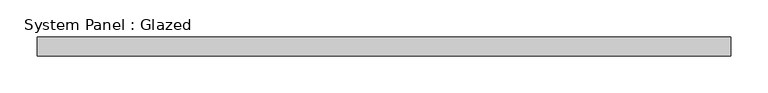
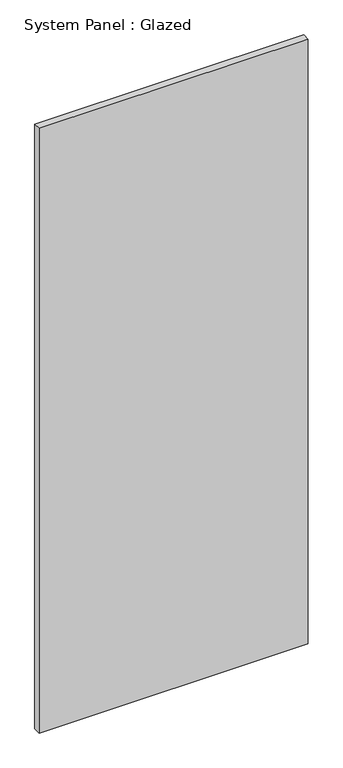
"""IFC4 building model written with IfcOpenShell, lengths in millimetres: plate geometry, System Panel : Glazed."""

import ifcopenshell
import ifcopenshell.guid

model = None  # the IFC model being written
_history = None  # IfcOwnerHistory: only IFC2X3 demands one
_inside = {}  # id of a spatial element -> (the spatial element, [elements in it])
_under = {}  # id of a project, library or spatial element -> (it, [spatial elements below it])
_declared = {}  # id of a project -> (the project, [libraries it declares])
_typed = {}  # id of a type object -> (the type object, [elements of that type])
_made_of = {}  # id of a material, layer set ... -> (it, [elements and type objects made of it])


def new_model(schema):
    """Start an empty IFC model of exactly this schema.

    Asked for "IFC4X3", IfcOpenShell would pick the latest addendum, in which some entities
    have other attributes; the version numbers below select the first issue.
    IFC2X3 requires an IfcOwnerHistory on every rooted entity: one is made here for all.
    """
    global model, _history
    if schema == "IFC4X3":
        model = ifcopenshell.file(schema_version=(4, 3, 0, 0))
    else:
        model = ifcopenshell.file(schema=schema)
    _inside.clear()
    _under.clear()
    _declared.clear()
    _typed.clear()
    _made_of.clear()
    _history = None
    if model.schema == "IFC2X3":
        org = make("IfcOrganization", Name="unknown")
        user = make(
            "IfcPersonAndOrganization",
            ThePerson=make("IfcPerson", FamilyName="unknown"),
            TheOrganization=org,
        )
        app = make(
            "IfcApplication",
            ApplicationDeveloper=org,
            Version="unknown",
            ApplicationFullName="unknown",
            ApplicationIdentifier="unknown",
        )
        _history = make(
            "IfcOwnerHistory",
            OwningUser=user,
            OwningApplication=app,
            ChangeAction="ADDED",
            CreationDate=0,
        )
    return model


def make(cls, **values):
    """One entity of the class cls with the attributes given. An attribute that is None is left unset."""
    return model.create_entity(
        cls, **{name: value for name, value in values.items() if value is not None}
    )


def rooted(cls, **values):
    """An entity with a GlobalId (a new one), such as an element, a storey or a relation."""
    return make(cls, GlobalId=ifcopenshell.guid.new(), OwnerHistory=_history, **values)


def si_unit(unit_type, name, prefix=None):
    """IfcSIUnit, for example si_unit("LENGTHUNIT", "METRE", prefix="MILLI")."""
    return make("IfcSIUnit", UnitType=unit_type, Prefix=prefix, Name=name)


def assignment(units):
    """IfcUnitAssignment: the units of a project."""
    return None if units is None else make("IfcUnitAssignment", Units=units)


def point(xyz):
    """IfcCartesianPoint."""
    return None if xyz is None else make("IfcCartesianPoint", Coordinates=xyz)


def direction(xyz):
    """IfcDirection."""
    return None if xyz is None else make("IfcDirection", DirectionRatios=xyz)


def frame(location, z_axis=None, x_axis=None):
    """IfcAxis2Placement3D, a coordinate frame: its origin and axes. An axis left out is left unset."""
    return make(
        "IfcAxis2Placement3D",
        Location=point(location),
        Axis=direction(z_axis),
        RefDirection=direction(x_axis),
    )


def origin():
    """The frame at (0, 0, 0) with its axes left unset."""
    return frame((0.0, 0.0, 0.0))


def origin_with_axes():
    """The frame at (0, 0, 0) with the z axis (0, 0, 1) and the x axis (1, 0, 0) written out."""
    return frame((0.0, 0.0, 0.0), z_axis=(0.0, 0.0, 1.0), x_axis=(1.0, 0.0, 0.0))


def place(relative_to, where):
    """IfcLocalPlacement: puts the frame where relative to a parent placement (None: the world)."""
    return make(
        "IfcLocalPlacement", PlacementRelTo=relative_to, RelativePlacement=where
    )


def context(
    kind, dimensions, precision=None, world=None, true_north=None, identifier=None
):
    """IfcGeometricRepresentationContext, for example the 3D "Model" context."""
    return make(
        "IfcGeometricRepresentationContext",
        ContextIdentifier=identifier,
        ContextType=kind,
        CoordinateSpaceDimension=dimensions,
        Precision=precision,
        WorldCoordinateSystem=world,
        TrueNorth=true_north,
    )


def project(units=None, contexts=None):
    """IfcProject with its units and contexts."""
    return rooted(
        "IfcProject",
        Name="project",
        RepresentationContexts=contexts,
        UnitsInContext=assignment(units),
    )


def spatial(cls, under=None, at=None, **own):
    """A site, building, storey or space (cls), placed at a placement, below another one or the project."""
    s = rooted(cls, ObjectPlacement=at, **own)
    if under is not None:
        _under.setdefault(under.id(), (under, []))[1].append(s)
    return s


def polyline(points):
    """IfcPolyline through the points."""
    return make("IfcPolyline", Points=[point(p) for p in points])


def outline(outer, holes=None, kind="AREA"):
    """IfcArbitraryClosedProfileDef: a profile drawn as a closed curve; with holes, ...WithVoids."""
    if holes is None:
        return make("IfcArbitraryClosedProfileDef", ProfileType=kind, OuterCurve=outer)
    return make(
        "IfcArbitraryProfileDefWithVoids",
        ProfileType=kind,
        OuterCurve=outer,
        InnerCurves=holes,
    )


def extrude(swept, where, along, depth):
    """IfcExtrudedAreaSolid: the profile swept, set in the frame where, extruded along a direction by depth."""
    return make(
        "IfcExtrudedAreaSolid",
        SweptArea=swept,
        Position=where,
        ExtrudedDirection=direction(along),
        Depth=depth,
    )


def shape(context_of_items, identifier, shape_type, items):
    """IfcShapeRepresentation: the items that make up one representation, for example the "Body"."""
    return make(
        "IfcShapeRepresentation",
        ContextOfItems=context_of_items,
        RepresentationIdentifier=identifier,
        RepresentationType=shape_type,
        Items=items,
    )


def source(mapping_origin, context_of_items, identifier, shape_type, items):
    """IfcRepresentationMap: a shape defined once, which mapped items show again and again."""
    return make(
        "IfcRepresentationMap",
        MappingOrigin=mapping_origin,
        MappedRepresentation=shape(context_of_items, identifier, shape_type, items),
    )


def transform(
    local_origin,
    x_axis=None,
    y_axis=None,
    z_axis=None,
    scale=None,
    scale2=None,
    scale3=None,
    uniform=True,
):
    """IfcCartesianTransformationOperator3D, or its non-uniform kind. x_axis, y_axis, z_axis: its Axis1, 2, 3."""
    if uniform:
        return make(
            "IfcCartesianTransformationOperator3D",
            Axis1=direction(x_axis),
            Axis2=direction(y_axis),
            LocalOrigin=point(local_origin),
            Scale=scale,
            Axis3=direction(z_axis),
        )
    return make(
        "IfcCartesianTransformationOperator3DnonUniform",
        Axis1=direction(x_axis),
        Axis2=direction(y_axis),
        LocalOrigin=point(local_origin),
        Scale=scale,
        Axis3=direction(z_axis),
        Scale2=scale2,
        Scale3=scale3,
    )


def mapped(mapping_source, mapping_target):
    """IfcMappedItem: shows the shape of a source again, moved by a transform."""
    return make(
        "IfcMappedItem", MappingSource=mapping_source, MappingTarget=mapping_target
    )


def made_of(thing, what):
    """Note that an element or type object is made of a material, layer set ...; save() writes the relation."""
    if what is not None:
        _made_of.setdefault(what.id(), (what, []))[1].append(thing)
    return thing


def element(
    cls,
    number,
    at=None,
    inside=None,
    cuts=None,
    type_object=None,
    material=None,
    context=None,
    identifier="Body",
    shape_type=None,
    held_by="IfcProductDefinitionShape",
    body=None,
    shapes=None,
    **own,
):
    """One element of the class cls, such as IfcWall. Its Tag is "e" and its number.

    at: its placement. inside: the storey or other place that contains it. cuts: it is an
    opening in that element (IfcRelVoidsElement). A single representation is given by context,
    identifier, shape_type and body (its items); several are given by shapes. held_by: the class
    of the entity that holds the representations. save() writes the other relations.
    """
    e = rooted(cls, Tag="e%d" % number, ObjectPlacement=at, **own)
    if body is not None:
        shapes = [shape(context, identifier, shape_type, body)]
    if shapes is not None:
        e.Representation = make(held_by, Representations=shapes)
    if inside is not None:
        _inside.setdefault(inside.id(), (inside, []))[1].append(e)
    if cuts is not None:
        rooted(
            "IfcRelVoidsElement", RelatingBuildingElement=cuts, RelatedOpeningElement=e
        )
    if type_object is not None:
        _typed.setdefault(type_object.id(), (type_object, []))[1].append(e)
    return made_of(e, material)


def aggregate(whole, parts):
    """IfcRelAggregates: a whole, such as a stair, and the parts it consists of."""
    return rooted("IfcRelAggregates", RelatingObject=whole, RelatedObjects=parts)


def save(model, path):
    """Write the relations noted so far, then the file.

    IfcRelAggregates (storeys below a building ...), IfcRelContainedInSpatialStructure (elements
    in a storey), IfcRelDefinesByType, IfcRelAssociatesMaterial and IfcRelDeclares: one each for
    every whole, place, type object, material and project.
    """
    for whole, parts in _under.values():
        aggregate(whole, parts)
    for where, things in _inside.values():
        rooted(
            "IfcRelContainedInSpatialStructure",
            RelatedElements=things,
            RelatingStructure=where,
        )
    for kind, things in _typed.values():
        rooted("IfcRelDefinesByType", RelatedObjects=things, RelatingType=kind)
    for what, things in _made_of.values():
        rooted("IfcRelAssociatesMaterial", RelatedObjects=things, RelatingMaterial=what)
    for by, libraries in _declared.values():
        rooted("IfcRelDeclares", RelatingContext=by, RelatedDefinitions=libraries)
    model.write(path)


def system_panel_glazed_c3e5734e(model_context):
    return source(origin(), model_context, "Body", "SweptSolid", [
        extrude(outline(polyline([(466.7250001, -44.45), (-466.7250001, -44.45), (-466.7250001, -19.05), (466.7250001, -19.05), (466.7250001, -44.45)])), origin_with_axes(), (0.0, 0.0, 1.0), 2216.15),
    ])


if __name__ == "__main__":
    model = new_model("IFC4")
    model_context = context("Model", 3, world=origin())
    ifc_project = project(units=[si_unit("LENGTHUNIT", "METRE", prefix="MILLI")], contexts=[model_context])
    site = spatial("IfcSite", under=ifc_project)
    building = spatial("IfcBuilding", under=site)
    placement = place(None, origin())
    system_panel_glazed_shape = system_panel_glazed_c3e5734e(model_context)
    element("IfcPlate", 1, ObjectType="System Panel : Glazed", at=placement, inside=building, context=model_context, shape_type="MappedRepresentation", body=[
        mapped(system_panel_glazed_shape, transform((0.0, 0.0, 0.0), x_axis=(1.0, 0.0, 0.0), y_axis=(0.0, 1.0, 0.0), z_axis=(0.0, 0.0, 1.0))),
    ])
    save(model, "model.ifc")

# Revit data of these elements
# Type "System Panel : Glazed"
#   Construction Type Id = "GSP4R"
#   Analytic Construction = "1/8 in Pilkington single glazing"
#   Visual Light Transmittance = 0.9
#   Solar Heat Gain Coefficient = 0.86
#   Heat Transfer Coefficient (U) = 1.18115 BTU/(h·ft²·°F)
#   Define Thermal Properties by = 1
# Element 1 (IfcPlate, "System Panel : Glazed")
#   Materials on its faces: "Glass"
# Materials
#   "Glass": class "Glass", colour RGB 0 128 192, transparency 0.75, Description = "Soda Lime Glass", Cost = 0
